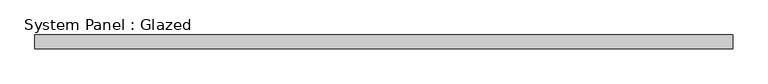
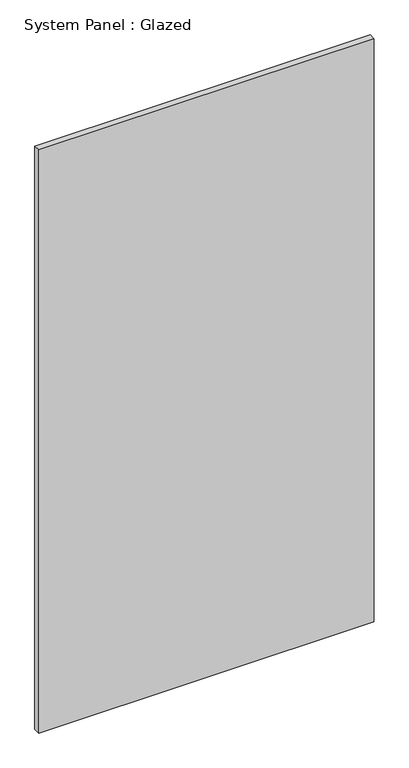
"""IFC4 building model written with IfcOpenShell, lengths in millimetres: plate geometry, System Panel : Glazed."""

import ifcopenshell
import ifcopenshell.guid

model = None  # the IFC model being written
_history = None  # IfcOwnerHistory: only IFC2X3 demands one
_inside = {}  # id of a spatial element -> (the spatial element, [elements in it])
_under = {}  # id of a project, library or spatial element -> (it, [spatial elements below it])
_declared = {}  # id of a project -> (the project, [libraries it declares])
_typed = {}  # id of a type object -> (the type object, [elements of that type])
_made_of = {}  # id of a material, layer set ... -> (it, [elements and type objects made of it])


def new_model(schema):
    """Start an empty IFC model of exactly this schema.

    Asked for "IFC4X3", IfcOpenShell would pick the latest addendum, in which some entities
    have other attributes; the version numbers below select the first issue.
    IFC2X3 requires an IfcOwnerHistory on every rooted entity: one is made here for all.
    """
    global model, _history
    if schema == "IFC4X3":
        model = ifcopenshell.file(schema_version=(4, 3, 0, 0))
    else:
        model = ifcopenshell.file(schema=schema)
    _inside.clear()
    _under.clear()
    _declared.clear()
    _typed.clear()
    _made_of.clear()
    _history = None
    if model.schema == "IFC2X3":
        org = make("IfcOrganization", Name="unknown")
        user = make(
            "IfcPersonAndOrganization",
            ThePerson=make("IfcPerson", FamilyName="unknown"),
            TheOrganization=org,
        )
        app = make(
            "IfcApplication",
            ApplicationDeveloper=org,
            Version="unknown",
            ApplicationFullName="unknown",
            ApplicationIdentifier="unknown",
        )
        _history = make(
            "IfcOwnerHistory",
            OwningUser=user,
            OwningApplication=app,
            ChangeAction="ADDED",
            CreationDate=0,
        )
    return model


def make(cls, **values):
    """One entity of the class cls with the attributes given. An attribute that is None is left unset."""
    return model.create_entity(
        cls, **{name: value for name, value in values.items() if value is not None}
    )


def rooted(cls, **values):
    """An entity with a GlobalId (a new one), such as an element, a storey or a relation."""
    return make(cls, GlobalId=ifcopenshell.guid.new(), OwnerHistory=_history, **values)


def si_unit(unit_type, name, prefix=None):
    """IfcSIUnit, for example si_unit("LENGTHUNIT", "METRE", prefix="MILLI")."""
    return make("IfcSIUnit", UnitType=unit_type, Prefix=prefix, Name=name)


def assignment(units):
    """IfcUnitAssignment: the units of a project."""
    return None if units is None else make("IfcUnitAssignment", Units=units)


def point(xyz):
    """IfcCartesianPoint."""
    return None if xyz is None else make("IfcCartesianPoint", Coordinates=xyz)


def direction(xyz):
    """IfcDirection."""
    return None if xyz is None else make("IfcDirection", DirectionRatios=xyz)


def frame(location, z_axis=None, x_axis=None):
    """IfcAxis2Placement3D, a coordinate frame: its origin and axes. An axis left out is left unset."""
    return make(
        "IfcAxis2Placement3D",
        Location=point(location),
        Axis=direction(z_axis),
        RefDirection=direction(x_axis),
    )


def origin():
    """The frame at (0, 0, 0) with its axes left unset."""
    return frame((0.0, 0.0, 0.0))


def origin_with_axes():
    """The frame at (0, 0, 0) with the z axis (0, 0, 1) and the x axis (1, 0, 0) written out."""
    return frame((0.0, 0.0, 0.0), z_axis=(0.0, 0.0, 1.0), x_axis=(1.0, 0.0, 0.0))


def place(relative_to, where):
    """IfcLocalPlacement: puts the frame where relative to a parent placement (None: the world)."""
    return make(
        "IfcLocalPlacement", PlacementRelTo=relative_to, RelativePlacement=where
    )


def context(
    kind, dimensions, precision=None, world=None, true_north=None, identifier=None
):
    """IfcGeometricRepresentationContext, for example the 3D "Model" context."""
    return make(
        "IfcGeometricRepresentationContext",
        ContextIdentifier=identifier,
        ContextType=kind,
        CoordinateSpaceDimension=dimensions,
        Precision=precision,
        WorldCoordinateSystem=world,
        TrueNorth=true_north,
    )


def project(units=None, contexts=None):
    """IfcProject with its units and contexts."""
    return rooted(
        "IfcProject",
        Name="project",
        RepresentationContexts=contexts,
        UnitsInContext=assignment(units),
    )


def spatial(cls, under=None, at=None, **own):
    """A site, building, storey or space (cls), placed at a placement, below another one or the project."""
    s = rooted(cls, ObjectPlacement=at, **own)
    if under is not None:
        _under.setdefault(under.id(), (under, []))[1].append(s)
    return s


def polyline(points):
    """IfcPolyline through the points."""
    return make("IfcPolyline", Points=[point(p) for p in points])


def outline(outer, holes=None, kind="AREA"):
    """IfcArbitraryClosedProfileDef: a profile drawn as a closed curve; with holes, ...WithVoids."""
    if holes is None:
        return make("IfcArbitraryClosedProfileDef", ProfileType=kind, OuterCurve=outer)
    return make(
        "IfcArbitraryProfileDefWithVoids",
        ProfileType=kind,
        OuterCurve=outer,
        InnerCurves=holes,
    )


def extrude(swept, where, along, depth):
    """IfcExtrudedAreaSolid: the profile swept, set in the frame where, extruded along a direction by depth."""
    return make(
        "IfcExtrudedAreaSolid",
        SweptArea=swept,
        Position=where,
        ExtrudedDirection=direction(along),
        Depth=depth,
    )


def shape(context_of_items, identifier, shape_type, items):
    """IfcShapeRepresentation: the items that make up one representation, for example the "Body"."""
    return make(
        "IfcShapeRepresentation",
        ContextOfItems=context_of_items,
        RepresentationIdentifier=identifier,
        RepresentationType=shape_type,
        Items=items,
    )


def source(mapping_origin, context_of_items, identifier, shape_type, items):
    """IfcRepresentationMap: a shape defined once, which mapped items show again and again."""
    return make(
        "IfcRepresentationMap",
        MappingOrigin=mapping_origin,
        MappedRepresentation=shape(context_of_items, identifier, shape_type, items),
    )


def transform(
    local_origin,
    x_axis=None,
    y_axis=None,
    z_axis=None,
    scale=None,
    scale2=None,
    scale3=None,
    uniform=True,
):
    """IfcCartesianTransformationOperator3D, or its non-uniform kind. x_axis, y_axis, z_axis: its Axis1, 2, 3."""
    if uniform:
        return make(
            "IfcCartesianTransformationOperator3D",
            Axis1=direction(x_axis),
            Axis2=direction(y_axis),
            LocalOrigin=point(local_origin),
            Scale=scale,
            Axis3=direction(z_axis),
        )
    return make(
        "IfcCartesianTransformationOperator3DnonUniform",
        Axis1=direction(x_axis),
        Axis2=direction(y_axis),
        LocalOrigin=point(local_origin),
        Scale=scale,
        Axis3=direction(z_axis),
        Scale2=scale2,
        Scale3=scale3,
    )


def mapped(mapping_source, mapping_target):
    """IfcMappedItem: shows the shape of a source again, moved by a transform."""
    return make(
        "IfcMappedItem", MappingSource=mapping_source, MappingTarget=mapping_target
    )


def made_of(thing, what):
    """Note that an element or type object is made of a material, layer set ...; save() writes the relation."""
    if what is not None:
        _made_of.setdefault(what.id(), (what, []))[1].append(thing)
    return thing


def element(
    cls,
    number,
    at=None,
    inside=None,
    cuts=None,
    type_object=None,
    material=None,
    context=None,
    identifier="Body",
    shape_type=None,
    held_by="IfcProductDefinitionShape",
    body=None,
    shapes=None,
    **own,
):
    """One element of the class cls, such as IfcWall. Its Tag is "e" and its number.

    at: its placement. inside: the storey or other place that contains it. cuts: it is an
    opening in that element (IfcRelVoidsElement). A single representation is given by context,
    identifier, shape_type and body (its items); several are given by shapes. held_by: the class
    of the entity that holds the representations. save() writes the other relations.
    """
    e = rooted(cls, Tag="e%d" % number, ObjectPlacement=at, **own)
    if body is not None:
        shapes = [shape(context, identifier, shape_type, body)]
    if shapes is not None:
        e.Representation = make(held_by, Representations=shapes)
    if inside is not None:
        _inside.setdefault(inside.id(), (inside, []))[1].append(e)
    if cuts is not None:
        rooted(
            "IfcRelVoidsElement", RelatingBuildingElement=cuts, RelatedOpeningElement=e
        )
    if type_object is not None:
        _typed.setdefault(type_object.id(), (type_object, []))[1].append(e)
    return made_of(e, material)


def aggregate(whole, parts):
    """IfcRelAggregates: a whole, such as a stair, and the parts it consists of."""
    return rooted("IfcRelAggregates", RelatingObject=whole, RelatedObjects=parts)


def save(model, path):
    """Write the relations noted so far, then the file.

    IfcRelAggregates (storeys below a building ...), IfcRelContainedInSpatialStructure (elements
    in a storey), IfcRelDefinesByType, IfcRelAssociatesMaterial and IfcRelDeclares: one each for
    every whole, place, type object, material and project.
    """
    for whole, parts in _under.values():
        aggregate(whole, parts)
    for where, things in _inside.values():
        rooted(
            "IfcRelContainedInSpatialStructure",
            RelatedElements=things,
            RelatingStructure=where,
        )
    for kind, things in _typed.values():
        rooted("IfcRelDefinesByType", RelatedObjects=things, RelatingType=kind)
    for what, things in _made_of.values():
        rooted("IfcRelAssociatesMaterial", RelatedObjects=things, RelatingMaterial=what)
    for by, libraries in _declared.values():
        rooted("IfcRelDeclares", RelatingContext=by, RelatedDefinitions=libraries)
    model.write(path)


def system_panel_glazed_7be3c4b1(model_context):
    return source(origin(), model_context, "Body", "SweptSolid", [
        extrude(outline(polyline([(633.0541355, 24.5), (-633.0541355, 24.5), (-633.0541355, 49.5), (633.0541355, 49.5), (633.0541355, 24.5)])), origin_with_axes(), (0.0, 0.0, 1.0), 2325.0),
    ])


if __name__ == "__main__":
    model = new_model("IFC4")
    model_context = context("Model", 3, world=origin())
    ifc_project = project(units=[si_unit("LENGTHUNIT", "METRE", prefix="MILLI")], contexts=[model_context])
    site = spatial("IfcSite", under=ifc_project)
    building = spatial("IfcBuilding", under=site)
    placement = place(None, origin())
    system_panel_glazed_shape = system_panel_glazed_7be3c4b1(model_context)
    element("IfcPlate", 1, ObjectType="System Panel : Glazed", at=placement, inside=building, context=model_context, shape_type="MappedRepresentation", body=[
        mapped(system_panel_glazed_shape, transform((0.0, 0.0, 0.0), x_axis=(1.0, 0.0, 0.0), y_axis=(0.0, 1.0, 0.0), z_axis=(0.0, 0.0, 1.0))),
    ])
    save(model, "model.ifc")

# Revit data of these elements
# Type "System Panel : Glazed"
#   Construction Type Id = "GSP4R"
#   Analytic Construction = "1/8 in Pilkington single glazing"
#   Visual Light Transmittance = 0.9
#   Solar Heat Gain Coefficient = 0.86
#   Heat Transfer Coefficient (U) = 6.7069 W/(m²·K)
#   Define Thermal Properties by = 1
# Element 1 (IfcPlate, "System Panel : Glazed")
#   Materials on its faces: "Glass"
# Materials
#   "Glass": class "Glass", colour RGB 0 128 192, transparency 0.9, Description = "Soda Lime Glass", Cost = 0
